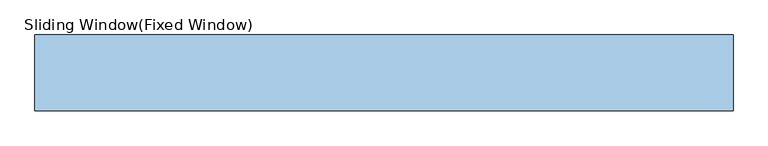
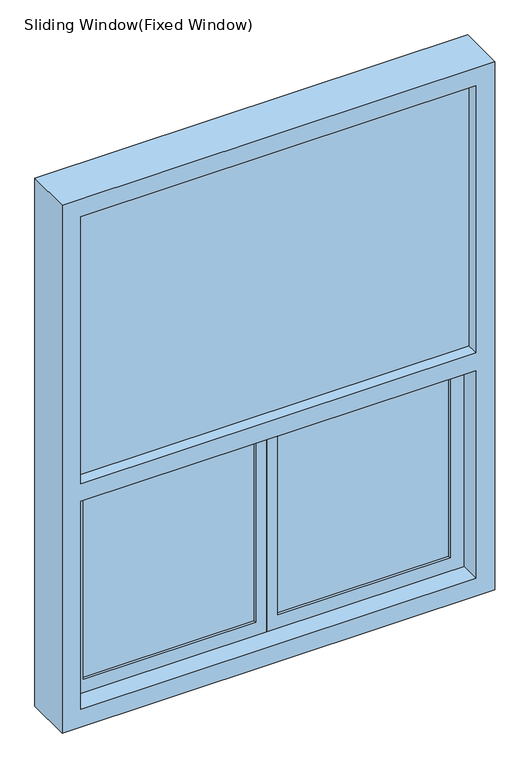
"""IFC4 building model written with IfcOpenShell, lengths in millimetres: window geometry, Sliding Window(Fixed Window) : H_WD_AR_B11_Fix_Sliding_Steel Window_DG_W1400xH1800_AW-1."""

from ifc_helpers import new_model, si_unit, frame, origin, place, context, project, spatial, polyline, outline, extrude, source, transform, mapped, element, save


def sliding_window_fixed_window_7f21aae4(model_context):
    return source(origin(), model_context, "Body", "SweptSolid", [
        extrude(outline(polyline([(2830.0, -690.0), (1050.0, -690.0), (1050.0, 690.0), (2830.0, 690.0), (2830.0, -690.0)]), holes=[polyline([(1810.0, 630.0), (1110.0, 630.0), (1110.0, -630.0), (1810.0, -630.0), (1810.0, 630.0)]), polyline([(1870.0, -630.0), (2770.0, -630.0), (2770.0, 630.0), (1870.0, 630.0), (1870.0, -630.0)])]), frame((0.0, -25.0, 0.0), z_axis=(0.0, 1.0, 0.0), x_axis=(0.0, 0.0, 1.0)), (0.0, 0.0, 1.0), 150.0),
        extrude(outline(polyline([(630.0, 37.0), (630.0, 13.0), (-630.0, 13.0), (-630.0, 37.0), (630.0, 37.0)])), frame((0.0, 0.0, 1870.0), z_axis=(0.0, 0.0, 1.0), x_axis=(1.0, 0.0, 0.0)), (0.0, 0.0, 1.0), 900.0),
        extrude(outline(polyline([(-35.0, 61.0), (-35.0, 49.0), (-585.0, 49.0), (-585.0, 61.0), (-35.0, 61.0)])), frame((0.0, 0.0, 1155.0), z_axis=(0.0, 0.0, 1.0), x_axis=(1.0, 0.0, 0.0)), (0.0, 0.0, 1.0), 610.0),
        extrude(outline(polyline([(1810.0, -630.0), (1110.0, -630.0), (1110.0, 0.0), (1810.0, 0.0), (1810.0, -630.0)]), holes=[polyline([(1765.0, -585.0), (1765.0, -35.0), (1155.0, -35.0), (1155.0, -585.0), (1765.0, -585.0)])]), frame((0.0, 40.0, 0.0), z_axis=(0.0, 1.0, 0.0), x_axis=(0.0, 0.0, 1.0)), (0.0, 0.0, 1.0), 30.0),
        extrude(outline(polyline([(585.0, 61.0), (585.0, 49.0), (35.0, 49.0), (35.0, 61.0), (585.0, 61.0)])), frame((0.0, 0.0, 1155.0), z_axis=(0.0, 0.0, 1.0), x_axis=(1.0, 0.0, 0.0)), (0.0, 0.0, 1.0), 610.0),
        extrude(outline(polyline([(1810.0, 0.0), (1110.0, 0.0), (1110.0, 630.0), (1810.0, 630.0), (1810.0, 0.0)]), holes=[polyline([(1765.0, 35.0), (1765.0, 585.0), (1155.0, 585.0), (1155.0, 35.0), (1765.0, 35.0)])]), frame((0.0, 40.0, 0.0), z_axis=(0.0, 1.0, 0.0), x_axis=(0.0, 0.0, 1.0)), (0.0, 0.0, 1.0), 30.0),
    ])


if __name__ == "__main__":
    model = new_model("IFC4")
    model_context = context("Model", 3, world=origin())
    ifc_project = project(units=[si_unit("LENGTHUNIT", "METRE", prefix="MILLI")], contexts=[model_context])
    site = spatial("IfcSite", under=ifc_project)
    building = spatial("IfcBuilding", under=site)
    placement = place(None, origin())
    sliding_window_fixed_window_shape = sliding_window_fixed_window_7f21aae4(model_context)
    element("IfcWindow", 1, ObjectType="Sliding Window(Fixed Window) : H_WD_AR_B11_Fix_Sliding_Steel Window_DG_W1400xH1800_AW-1", at=placement, inside=building, context=model_context, shape_type="MappedRepresentation", body=[
        mapped(sliding_window_fixed_window_shape, transform((0.0, 0.0, 0.0), x_axis=(1.0, 0.0, 0.0), y_axis=(0.0, 1.0, 0.0), z_axis=(0.0, 0.0, 1.0))),
    ])
    save(model, "model.ifc")

# Revit data of these elements
# Type "Sliding Window(Fixed Window) : H_WD_AR_B11_Fix_Sliding_Steel Window_DG_W1400xH1800_AW-1"
#   Type Mark = "268"
#   Analytic Construction = "<None>"
#   미서기창 높이 = 700 mm
#   Main Window = 1400 mm
#   Height = 1800 mm
#   Mullion Thk = 60 mm
#   Frame = 150 mm
#   Default Sill Height = 1040 mm
#   Width = 1400 mm
#   Define Thermal Properties by = 1
#   Wall Closure = (empty or 0)
# Element 1 (IfcWindow, "Sliding Window(Fixed Window) : H_WD_AR_B11_Fix_Sliding_Steel Window_DG_W1400xH1800_AW-1")
#   Materials on its faces: "00_Metal_Aluminum", "Glass"
# Materials
#   "00_Metal_Aluminum": class "Metal", colour RGB 244 244 244, transparency 0, Description = "Aluminum", Cost = 0, Image = none
#   "Glass": class "Glass", colour RGB 218 227 224, transparency 0.85, Description = "Soda Lime Glass", Cost = 0
